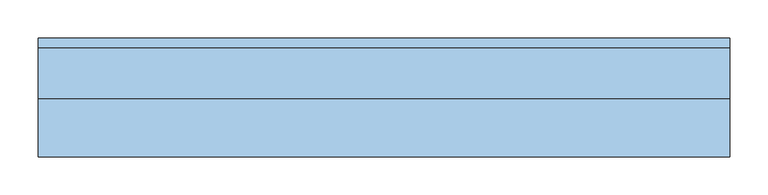
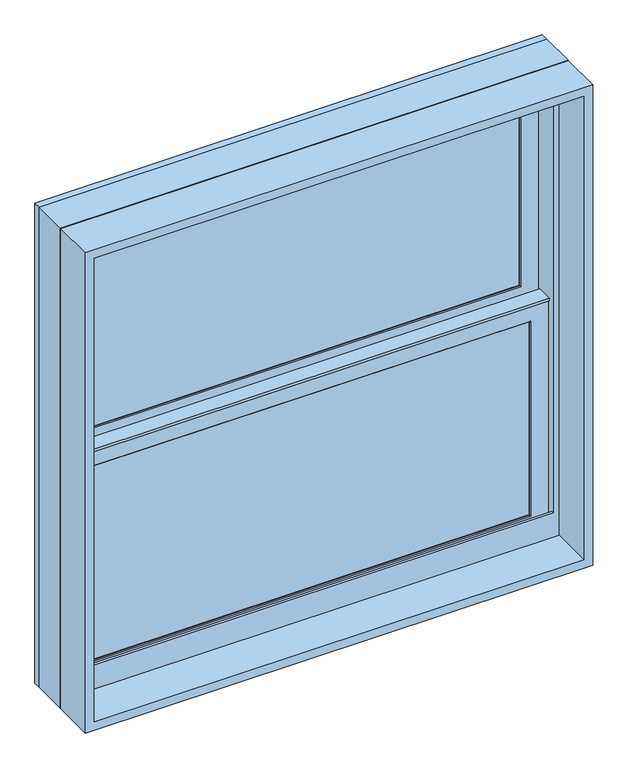
"""IFC4 building model written with IfcOpenShell, lengths in millimetres: window geometry, Window-Double_Hung-Marvin-Essential : ESDH3030."""

from ifc_helpers import new_model, si_unit, frame, origin, place, context, project, spatial, polyline, outline, extrude, faceted_brep, source, transform, mapped, element, save


def window_75fe73d6(model_context):
    return source(origin(), model_context, "Body", "SolidModel", [
        extrude(outline(polyline([(140.7583333, 20.6375), (140.7583333, 15.875), (121.7083333, 15.875), (121.7083333, 20.6375), (140.7583333, 20.6375)])), frame((0.0, 0.0, 1593.85), z_axis=(0.0, 0.0, 1.0), x_axis=(1.0, 0.0, 0.0)), (0.0, 0.0, 1.0), 374.65),
        extrude(outline(polyline([(-121.7083333, 20.6375), (-121.7083333, 15.875), (-140.7583333, 15.875), (-140.7583333, 20.6375), (-121.7083333, 20.6375)])), frame((0.0, 0.0, 1593.85), z_axis=(0.0, 0.0, 1.0), x_axis=(1.0, 0.0, 0.0)), (0.0, 0.0, 1.0), 374.65),
        extrude(outline(polyline([(393.7, 20.6375), (393.7, 15.875), (-393.7, 15.875), (-393.7, 20.6375), (393.7, 20.6375)])), frame((0.0, 0.0, 1771.65), z_axis=(0.0, 0.0, 1.0), x_axis=(1.0, 0.0, 0.0)), (0.0, 0.0, 1.0), 19.05),
        extrude(outline(polyline([(-140.7583333, 46.83125), (-140.7583333, 51.59375), (-121.7083333, 51.59375), (-121.7083333, 46.83125), (-140.7583333, 46.83125)])), frame((0.0, 0.0, 2006.6), z_axis=(0.0, 0.0, 1.0), x_axis=(1.0, 0.0, 0.0)), (0.0, 0.0, 1.0), 374.65),
        extrude(outline(polyline([(121.7083333, 46.83125), (121.7083333, 51.59375), (140.7583333, 51.59375), (140.7583333, 46.83125), (121.7083333, 46.83125)])), frame((0.0, 0.0, 2006.6), z_axis=(0.0, 0.0, 1.0), x_axis=(1.0, 0.0, 0.0)), (0.0, 0.0, 1.0), 374.65),
        extrude(outline(polyline([(-393.7, 46.83125), (-393.7, 51.59375), (393.7, 51.59375), (393.7, 46.83125), (-393.7, 46.83125)])), frame((0.0, 0.0, 2184.4), z_axis=(0.0, 0.0, 1.0), x_axis=(1.0, 0.0, 0.0)), (0.0, 0.0, 1.0), 19.05),
        extrude(outline(polyline([(140.7583333, 20.6375), (121.7083333, 20.6375), (121.7083333, 25.4), (140.7583333, 25.4), (140.7583333, 20.6375)])), frame((0.0, 0.0, 1593.85), z_axis=(0.0, 0.0, 1.0), x_axis=(1.0, 0.0, 0.0)), (0.0, 0.0, 1.0), 374.65),
        extrude(outline(polyline([(-121.7083333, 20.6375), (-140.7583333, 20.6375), (-140.7583333, 25.4), (-121.7083333, 25.4), (-121.7083333, 20.6375)])), frame((0.0, 0.0, 1593.85), z_axis=(0.0, 0.0, 1.0), x_axis=(1.0, 0.0, 0.0)), (0.0, 0.0, 1.0), 374.65),
        extrude(outline(polyline([(393.7, 20.6375), (-393.7, 20.6375), (-393.7, 25.4), (393.7, 25.4), (393.7, 20.6375)])), frame((0.0, 0.0, 1771.65), z_axis=(0.0, 0.0, 1.0), x_axis=(1.0, 0.0, 0.0)), (0.0, 0.0, 1.0), 19.05),
        extrude(outline(polyline([(-140.7583333, 56.35625), (-121.7083333, 56.35625), (-121.7083333, 51.59375), (-140.7583333, 51.59375), (-140.7583333, 56.35625)])), frame((0.0, 0.0, 2006.6), z_axis=(0.0, 0.0, 1.0), x_axis=(1.0, 0.0, 0.0)), (0.0, 0.0, 1.0), 374.65),
        extrude(outline(polyline([(121.7083333, 56.35625), (140.7583333, 56.35625), (140.7583333, 51.59375), (121.7083333, 51.59375), (121.7083333, 56.35625)])), frame((0.0, 0.0, 2006.6), z_axis=(0.0, 0.0, 1.0), x_axis=(1.0, 0.0, 0.0)), (0.0, 0.0, 1.0), 374.65),
        extrude(outline(polyline([(-393.7, 56.35625), (393.7, 56.35625), (393.7, 51.59375), (-393.7, 51.59375), (-393.7, 56.35625)])), frame((0.0, 0.0, 2184.4), z_axis=(0.0, 0.0, 1.0), x_axis=(1.0, 0.0, 0.0)), (0.0, 0.0, 1.0), 19.05),
        faceted_brep([(-420.6875, 5.6780605, 1998.5351748), (-420.6875, 5.6780605, 1993.9), (420.6875, 5.6780605, 1993.9), (420.6875, 5.6780605, 1998.5351748), (-420.6875, 34.8118605, 1998.5351748), (420.6875, 34.8118605, 1998.5351748), (420.6875, 34.8118605, 1993.9), (-420.6875, 34.8118605, 1993.9), (-420.6875, 30.1625, 1993.9), (-420.6875, 30.1625, 1566.8625), (-420.6875, 8.9241104, 1566.8625), (-420.6875, 8.9241104, 1993.9), (420.6875, 8.9241104, 1993.9), (420.6875, 30.1625, 1993.9), (420.6875, 8.9241104, 1566.8625), (420.6875, 30.1625, 1566.8625), (-404.8034752, 11.90625, 1979.6034752), (-404.8034752, 30.1625, 1979.6034752), (404.8034752, 30.1625, 1979.6034752), (404.8034752, 11.90625, 1979.6034752), (-388.14375, 10.4662439, 1962.94375), (-388.14375, 11.90625, 1962.94375), (388.14375, 11.90625, 1962.94375), (388.14375, 10.4662439, 1962.94375), (389.6858834, 8.9241104, 1964.4858834), (-389.6858834, 8.9241104, 1964.4858834), (404.8034752, 30.1625, 1582.7465248), (404.8034752, 11.90625, 1582.7465248), (388.14375, 11.90625, 1599.40625), (388.14375, 10.4662439, 1599.40625), (389.6858834, 8.9241104, 1597.8641166), (-404.8034752, 30.1625, 1582.7465248), (-404.8034752, 11.90625, 1582.7465248), (-388.14375, 11.90625, 1599.40625), (-388.14375, 10.4662439, 1599.40625), (-389.6858834, 8.9241104, 1597.8641166)], [[[0, 1, 2, 3]], [[4, 5, 6, 7]], [[1, 0, 4, 7, 8, 9, 10, 11]], [[2, 1, 11, 12]], [[7, 6, 13, 8]], [[3, 2, 12, 14, 15, 13, 6, 5]], [[0, 3, 5, 4]], [[16, 17, 18, 19]], [[20, 21, 22, 23]], [[20, 23, 24, 25]], [[19, 18, 26, 27]], [[23, 22, 28, 29]], [[24, 23, 29, 30]], [[27, 26, 31, 32]], [[29, 28, 33, 34]], [[30, 29, 34, 35]], [[15, 14, 10, 9]], [[15, 9, 8, 13], [18, 17, 31, 26]], [[17, 16, 32, 31]], [[16, 19, 27, 32], [22, 21, 33, 28]], [[21, 20, 34, 33]], [[20, 25, 35, 34]], [[10, 14, 12, 11], [25, 24, 30, 35]]]),
        extrude(outline(polyline([(38.5955581, 1979.6125), (33.5778968, 1979.6125), (33.5778968, 1981.2), (39.9405976, 1981.2), (39.9405976, 1979.6125), (61.515625, 1979.6125), (47.6307501, 1976.2975159), (38.5955581, 1976.2975159), (38.5955581, 1979.6125)])), frame((-420.6875, 0.0, 0.0), z_axis=(1.0, 0.0, 0.0), x_axis=(0.0, 1.0, 0.0)), (0.0, 0.0, 1.0), 841.375),
        faceted_brep([(450.85, 0.0, 1536.7), (450.85, 0.0, 2438.4), (-450.85, 0.0, 2438.4), (-450.85, 0.0, 1536.7), (424.65625, 0.0, 1597.81875), (-424.65625, 0.0, 1597.81875), (-424.65625, 0.0, 2412.20625), (424.65625, 0.0, 2412.20625), (424.65625, 3.96875, 1536.7), (-424.65625, 3.96875, 1536.7), (-424.65625, 3.96875, 1597.81875), (424.65625, 3.96875, 1597.81875), (-450.85, 65.6828125, 1536.7), (-424.65625, 65.6828125, 1536.7), (424.65625, 65.6828125, 1536.7), (450.85, 65.6828125, 1536.7), (-450.85, 65.6828125, 2438.4), (450.85, 65.6828125, 2438.4), (424.65625, 65.6828125, 2412.20625), (-424.65625, 65.6828125, 2412.20625)], [[[0, 1, 2, 3], [4, 5, 6, 7]], [[8, 9, 10, 11]], [[5, 4, 11, 10]], [[0, 3, 12, 13, 9, 8, 14, 15]], [[13, 12, 16, 17, 15, 14, 18, 19]], [[13, 19, 6, 5, 10, 9]], [[7, 6, 19, 18]], [[18, 14, 8, 11, 4, 7]], [[1, 0, 15, 17]], [[2, 1, 17, 16]], [[3, 2, 16, 12]]]),
        faceted_brep([(424.65625, 30.1625, 1987.55), (423.06875, 30.1625, 1987.55), (423.06875, 30.1625, 1561.0544613), (424.65625, 30.1625, 1561.0544613), (-423.06875, 30.1625, 1987.55), (-424.65625, 30.1625, 1987.55), (-424.65625, 30.1625, 1561.0544613), (-423.06875, 30.1625, 1561.0544613), (423.06875, 63.5, 1987.55), (424.65625, 63.5, 1987.55), (424.65625, 63.5, 1554.5743077), (423.06875, 63.5, 1554.5743077), (-424.65625, 63.5, 1987.55), (-423.06875, 63.5, 1987.55), (-423.06875, 63.5, 1554.5743077), (-424.65625, 63.5, 1554.5743077), (435.9108932, 3.96875, 1566.1460105), (435.9108932, 3.96875, 1536.7), (435.9108932, 65.6828125, 1536.7), (435.9108932, 65.6828125, 1554.150012), (-435.9108932, 3.96875, 1536.7), (-435.9108932, 3.96875, 1566.1460105), (-435.9108932, 65.6828125, 1554.150012), (-435.9108932, 65.6828125, 1536.7), (435.9108932, 78.58125, 1551.6428097), (-435.9108932, 78.58125, 1551.6428097), (-433.8971252, 68.2348864, 1553.6539391), (-415.93135, 68.2348864, 1553.6539391), (-415.93135, 65.6828125, 1554.150012), (415.93135, 65.6828125, 1554.150012), (415.93135, 68.2348864, 1553.6539391), (433.8971252, 68.2348864, 1553.6539391), (-450.85, 65.6828125, 1536.7), (-450.85, 78.5948249, 1536.7), (450.85, 78.5948249, 1536.7), (450.85, 65.6828125, 1536.7), (-450.85, 78.58125, 2438.4), (450.85, 78.58125, 2438.4), (435.9108932, 78.58125, 2423.4608932), (-435.9108932, 78.58125, 2423.4608932), (-450.85, 65.6828125, 2438.4), (-433.8971252, 68.2348864, 2421.4471252), (433.8971252, 68.2348864, 2421.4471252), (415.93135, 68.2348864, 2403.48135), (-415.93135, 68.2348864, 2403.48135), (-415.93135, 65.6828125, 2403.48135), (415.93135, 65.6828125, 2403.48135), (450.85, 65.6828125, 2438.4)], [[[0, 1, 2, 3]], [[4, 5, 6, 7]], [[8, 9, 10, 11]], [[12, 13, 14, 15]], [[1, 8, 11, 2]], [[9, 0, 3, 10]], [[1, 0, 9, 8]], [[5, 4, 13, 12]], [[5, 12, 15, 6]], [[13, 4, 7, 14]], [[16, 17, 18, 19]], [[20, 21, 22, 23]], [[24, 25, 26, 27, 28, 22, 21, 16, 19, 29, 30, 31], [3, 2, 11, 10], [7, 6, 15, 14]], [[17, 16, 21, 20]], [[17, 20, 23, 32, 33, 34, 35, 18]], [[34, 33, 36, 37], [25, 24, 38, 39]], [[33, 32, 40, 36]], [[39, 41, 26, 25]], [[41, 42, 31, 30, 43, 44, 27, 26]], [[44, 45, 28, 27]], [[40, 32, 23, 22, 28, 45, 46, 29, 19, 18, 35, 47]], [[36, 40, 47, 37]], [[39, 38, 42, 41]], [[44, 43, 46, 45]], [[34, 37, 47, 35]], [[42, 38, 24, 31]], [[46, 43, 30, 29]]]),
        extrude(outline(polyline([(400.84375, 11.90625), (-400.84375, 11.90625), (-400.84375, 15.08125), (400.84375, 15.08125), (400.84375, 11.90625)])), frame((0.0, 0.0, 1586.70625), z_axis=(0.0, 0.0, 1.0), x_axis=(1.0, 0.0, 0.0)), (0.0, 0.0, 1.0), 388.9375),
        extrude(outline(polyline([(400.84375, 42.8625), (-400.84375, 42.8625), (-400.84375, 46.0375), (400.84375, 46.0375), (400.84375, 42.8625)])), frame((0.0, 0.0, 1999.45625), z_axis=(0.0, 0.0, 1.0), x_axis=(1.0, 0.0, 0.0)), (0.0, 0.0, 1.0), 388.9375),
        faceted_brep([(-388.14375, 31.194477, 1962.94375), (-389.6858834, 32.7366104, 1964.4858834), (389.6858834, 32.7366104, 1964.4858834), (388.14375, 31.194477, 1962.94375), (-388.14375, 30.1625, 1962.94375), (388.14375, 30.1625, 1962.94375), (-420.6875, 32.7366104, 1995.4875), (-420.6875, 30.1625, 1995.4875), (420.6875, 30.1625, 1995.4875), (420.6875, 32.7366104, 1995.4875), (389.6858834, 32.7366104, 1597.8641166), (388.14375, 31.194477, 1599.40625), (388.14375, 30.1625, 1599.40625), (420.6875, 30.1625, 1566.8625), (420.6875, 32.7366104, 1566.8625), (-389.6858834, 32.7366104, 1597.8641166), (-388.14375, 31.194477, 1599.40625), (-388.14375, 30.1625, 1599.40625), (-420.6875, 30.1625, 1566.8625), (-420.6875, 32.7366104, 1566.8625)], [[[0, 1, 2, 3]], [[4, 0, 3, 5]], [[6, 7, 8, 9]], [[3, 2, 10, 11]], [[5, 3, 11, 12]], [[9, 8, 13, 14]], [[11, 10, 15, 16]], [[12, 11, 16, 17]], [[14, 13, 18, 19]], [[9, 14, 19, 6], [1, 15, 10, 2]], [[16, 15, 1, 0]], [[17, 16, 0, 4]], [[7, 18, 13, 8], [5, 12, 17, 4]], [[19, 18, 7, 6]]]),
        faceted_brep([(-404.8034752, 42.8625, 2392.3534752), (-404.8034752, 61.11875, 2392.3534752), (404.8034752, 61.11875, 2392.3534752), (404.8034752, 42.8625, 2392.3534752), (-388.14375, 41.4224939, 2375.69375), (-388.14375, 42.8625, 2375.69375), (388.14375, 42.8625, 2375.69375), (388.14375, 41.4224939, 2375.69375), (-389.6858834, 39.8803604, 2377.2358834), (389.6858834, 39.8803604, 2377.2358834), (-420.6875, 61.11875, 2408.2375), (-420.6875, 39.8803604, 2408.2375), (420.6875, 39.8803604, 2408.2375), (420.6875, 61.11875, 2408.2375), (404.8034752, 61.11875, 1995.4965248), (404.8034752, 42.8625, 1995.4965248), (388.14375, 42.8625, 2012.15625), (388.14375, 41.4224939, 2012.15625), (389.6858834, 39.8803604, 2010.6141166), (420.6875, 39.8803604, 1979.6125), (420.6875, 61.11875, 1979.6125), (-404.8034752, 61.11875, 1995.4965248), (-404.8034752, 42.8625, 1995.4965248), (-388.14375, 42.8625, 2012.15625), (-388.14375, 41.4224939, 2012.15625), (-389.6858834, 39.8803604, 2010.6141166), (-420.6875, 39.8803604, 1979.6125), (-420.6875, 61.11875, 1979.6125)], [[[0, 1, 2, 3]], [[4, 5, 6, 7]], [[8, 4, 7, 9]], [[10, 11, 12, 13]], [[3, 2, 14, 15]], [[7, 6, 16, 17]], [[9, 7, 17, 18]], [[13, 12, 19, 20]], [[15, 14, 21, 22]], [[17, 16, 23, 24]], [[18, 17, 24, 25]], [[20, 19, 26, 27]], [[13, 20, 27, 10], [1, 21, 14, 2]], [[22, 21, 1, 0]], [[3, 15, 22, 0], [5, 23, 16, 6]], [[24, 23, 5, 4]], [[25, 24, 4, 8]], [[11, 26, 19, 12], [9, 18, 25, 8]], [[27, 26, 11, 10]]]),
        faceted_brep([(-420.6875, 61.11875, 1979.6125), (-420.6875, 63.6928604, 1979.6125), (420.6875, 63.6928604, 1979.6125), (420.6875, 61.11875, 1979.6125), (-388.14375, 62.150727, 2012.15625), (-388.14375, 61.11875, 2012.15625), (388.14375, 61.11875, 2012.15625), (388.14375, 62.150727, 2012.15625), (-389.6858834, 63.6928604, 2010.6141166), (389.6858834, 63.6928604, 2010.6141166), (420.6875, 63.6928604, 2408.2375), (420.6875, 61.11875, 2408.2375), (388.14375, 61.11875, 2375.69375), (388.14375, 62.150727, 2375.69375), (389.6858834, 63.6928604, 2377.2358834), (-420.6875, 63.6928604, 2408.2375), (-420.6875, 61.11875, 2408.2375), (-388.14375, 61.11875, 2375.69375), (-388.14375, 62.150727, 2375.69375), (-389.6858834, 63.6928604, 2377.2358834)], [[[0, 1, 2, 3]], [[4, 5, 6, 7]], [[8, 4, 7, 9]], [[3, 2, 10, 11]], [[7, 6, 12, 13]], [[9, 7, 13, 14]], [[11, 10, 15, 16]], [[13, 12, 17, 18]], [[14, 13, 18, 19]], [[16, 15, 1, 0]], [[3, 11, 16, 0], [5, 17, 12, 6]], [[18, 17, 5, 4]], [[19, 18, 4, 8]], [[1, 15, 10, 2], [9, 14, 19, 8]]]),
        extrude(outline(polyline([(400.84375, 26.19375), (-400.84375, 26.19375), (-400.84375, 30.1625), (400.84375, 30.1625), (400.84375, 26.19375)])), frame((0.0, 0.0, 1586.70625), z_axis=(0.0, 0.0, 1.0), x_axis=(1.0, 0.0, 0.0)), (0.0, 0.0, 1.0), 388.9375),
        extrude(outline(polyline([(400.84375, 57.15), (-400.84375, 57.15), (-400.84375, 61.11875), (400.84375, 61.11875), (400.84375, 57.15)])), frame((0.0, 0.0, 1999.45625), z_axis=(0.0, 0.0, 1.0), x_axis=(1.0, 0.0, 0.0)), (0.0, 0.0, 1.0), 388.9375),
        extrude(outline(polyline([(2438.4, 450.85), (2438.4, -450.85), (1536.7, -450.85), (1536.7, 450.85), (2438.4, 450.85)]), holes=[polyline([(2422.525, 434.975), (1552.575, 434.975), (1552.575, -434.975), (2422.525, -434.975), (2422.525, 434.975)])]), frame((0.0, -76.2, 0.0), z_axis=(0.0, 1.0, 0.0), x_axis=(0.0, 0.0, 1.0)), (0.0, 0.0, 1.0), 75.40625),
    ])


if __name__ == "__main__":
    model = new_model("IFC4")
    model_context = context("Model", 3, world=origin())
    ifc_project = project(units=[si_unit("LENGTHUNIT", "METRE", prefix="MILLI")], contexts=[model_context])
    site = spatial("IfcSite", under=ifc_project)
    building = spatial("IfcBuilding", under=site)
    placement = place(None, origin())
    window_shape = window_75fe73d6(model_context)
    element("IfcWindow", 1, ObjectType="Window-Double_Hung-Marvin-Essential : ESDH3030", at=placement, inside=building, context=model_context, shape_type="MappedRepresentation", body=[
        mapped(window_shape, transform((0.0, 0.0, 0.0), x_axis=(1.0, 0.0, 0.0), y_axis=(0.0, 1.0, 0.0), z_axis=(0.0, 0.0, 1.0))),
    ])
    save(model, "model.ifc")

# Revit data of these elements
# Type "Window-Double_Hung-Marvin-Essential : ESDH3030"
#   Type Mark = "37"
#   Window Type = "Essential Double Hung"
#   Product data url = "https://bimobject.com/marvin-windows-and-doors/product/marvin-dhwau"
#   Product Guid = "c4a96547-874c-4385-91dc-a058adc19d98"
#   Frame = "All Ultrex"
#   Egress Window = "No"
#   URL = "www.marvin.com"
#   Model = "ESDH3030"
#   Manufacturer = "Marvin Windows and Doors"
#   Label Egress = ""
#   Glass Type = "IG Low E II with Argon"
#   Design Pressure = "DP50"
#   Description = "3636 DBHG"
#   Analytic Construction = "<None>"
#   Prairie Corner Width = 0' - 4"
#   Prairie Corner Height = 0' - 4"
#   Egress Width = 2' - 8 9/16"
#   Egress Height = 1' - 1 27/128"
#   Rough Width = 3' - 0"
#   Rough Height = 3' - 0"
#   Nominal Width = 3' - 0"
#   Nominal Height = 3' - 0"
#   Inset to Installation Flange [instance default] = 0' - 1"
#   Height = 2' - 11 1/2"
#   Egress Area = 2.98737 SF
#   Default Head Height = 8' - 0"
#   Width = 2' - 11 1/2"
#   Daylight Area = 6.07536 SF
#   DLO Width = 2' - 6 9/16"
#   DLO Height = 1' - 2 5/16"
#   Muntins Top Sash = yes
#   Lites Wide Top Sash = 3
#   Lites Wide Bottom Sash = 3
#   Lites High Top Sash = 2
#   Lites High Bottom Sash = 2
#   Lite Cut Prairie 9 = no
#   Lite Cut HV Grid = yes
#   Muntins Bottom Sash = yes
#   Label Visibility = no
#   Jamb Extension Visibility = yes
#   Edition number = 1
#   Interior Material = Ultrex-Marvin-Stonewhite
#   Glazing Material = Glass-Marvin-IG Low E II with Argon
#   Cladding Material = Ultrex-Marvin-Pebblegray
#   Wall Closure = (empty or 0)
#   Assembly Code = ""
# Element 1 (IfcWindow, "Window-Double_Hung-Marvin-Essential : ESDH3030")
#   Materials on its faces: "Ultrex-Marvin-Pebblegray", "Ultrex-Marvin-Stonewhite", "Glass-Marvin-IG Low E II with Argon"
# Materials
#   "Ultrex-Marvin-Stonewhite": class "Paint", colour RGB 250 251 245, transparency 0
#   "Glass-Marvin-IG Low E II with Argon": class "Glass", colour RGB 0 128 192, transparency 0.85
#   "Ultrex-Marvin-Pebblegray": class "Paint", colour RGB 189 185 173, transparency 0
